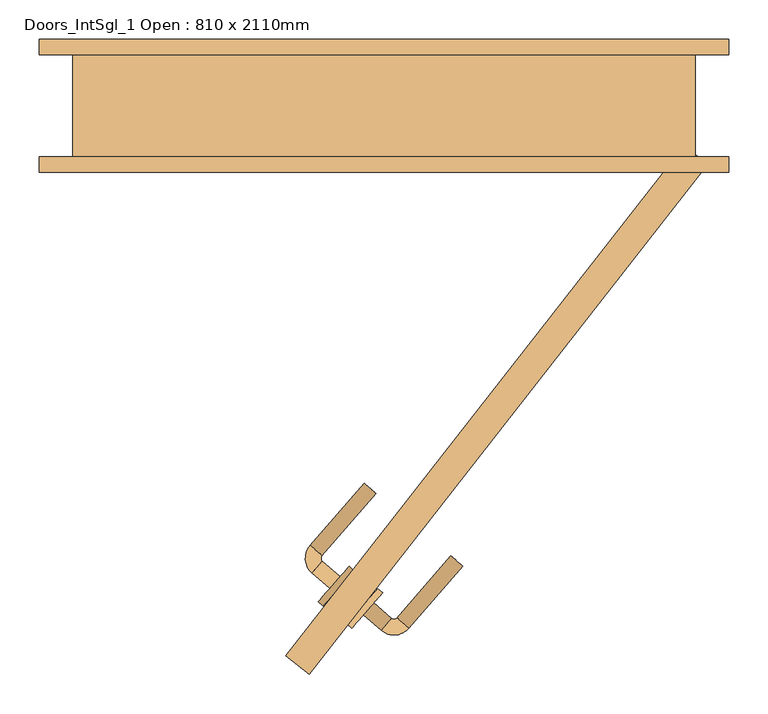
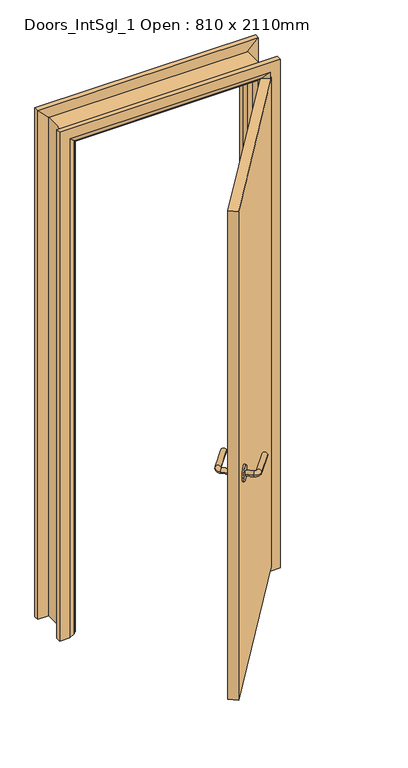
"""IFC4 building model written with IfcOpenShell, lengths in millimetres: door geometry, Doors_IntSgl_1 Open : 810 x 2110mm."""

import ifcopenshell
import ifcopenshell.guid

model = None  # the IFC model being written
_history = None  # IfcOwnerHistory: only IFC2X3 demands one
_inside = {}  # id of a spatial element -> (the spatial element, [elements in it])
_under = {}  # id of a project, library or spatial element -> (it, [spatial elements below it])
_declared = {}  # id of a project -> (the project, [libraries it declares])
_typed = {}  # id of a type object -> (the type object, [elements of that type])
_made_of = {}  # id of a material, layer set ... -> (it, [elements and type objects made of it])


def new_model(schema):
    """Start an empty IFC model of exactly this schema.

    Asked for "IFC4X3", IfcOpenShell would pick the latest addendum, in which some entities
    have other attributes; the version numbers below select the first issue.
    IFC2X3 requires an IfcOwnerHistory on every rooted entity: one is made here for all.
    """
    global model, _history
    if schema == "IFC4X3":
        model = ifcopenshell.file(schema_version=(4, 3, 0, 0))
    else:
        model = ifcopenshell.file(schema=schema)
    _inside.clear()
    _under.clear()
    _declared.clear()
    _typed.clear()
    _made_of.clear()
    _history = None
    if model.schema == "IFC2X3":
        org = make("IfcOrganization", Name="unknown")
        user = make(
            "IfcPersonAndOrganization",
            ThePerson=make("IfcPerson", FamilyName="unknown"),
            TheOrganization=org,
        )
        app = make(
            "IfcApplication",
            ApplicationDeveloper=org,
            Version="unknown",
            ApplicationFullName="unknown",
            ApplicationIdentifier="unknown",
        )
        _history = make(
            "IfcOwnerHistory",
            OwningUser=user,
            OwningApplication=app,
            ChangeAction="ADDED",
            CreationDate=0,
        )
    return model


def make(cls, **values):
    """One entity of the class cls with the attributes given. An attribute that is None is left unset."""
    return model.create_entity(
        cls, **{name: value for name, value in values.items() if value is not None}
    )


def rooted(cls, **values):
    """An entity with a GlobalId (a new one), such as an element, a storey or a relation."""
    return make(cls, GlobalId=ifcopenshell.guid.new(), OwnerHistory=_history, **values)


def si_unit(unit_type, name, prefix=None):
    """IfcSIUnit, for example si_unit("LENGTHUNIT", "METRE", prefix="MILLI")."""
    return make("IfcSIUnit", UnitType=unit_type, Prefix=prefix, Name=name)


def assignment(units):
    """IfcUnitAssignment: the units of a project."""
    return None if units is None else make("IfcUnitAssignment", Units=units)


def point(xyz):
    """IfcCartesianPoint."""
    return None if xyz is None else make("IfcCartesianPoint", Coordinates=xyz)


def direction(xyz):
    """IfcDirection."""
    return None if xyz is None else make("IfcDirection", DirectionRatios=xyz)


def frame(location, z_axis=None, x_axis=None):
    """IfcAxis2Placement3D, a coordinate frame: its origin and axes. An axis left out is left unset."""
    return make(
        "IfcAxis2Placement3D",
        Location=point(location),
        Axis=direction(z_axis),
        RefDirection=direction(x_axis),
    )


def frame_2d(location, x_axis=None):
    """IfcAxis2Placement2D, a coordinate frame in the plane: its origin and x axis."""
    return make(
        "IfcAxis2Placement2D", Location=point(location), RefDirection=direction(x_axis)
    )


def origin():
    """The frame at (0, 0, 0) with its axes left unset."""
    return frame((0.0, 0.0, 0.0))


def place(relative_to, where):
    """IfcLocalPlacement: puts the frame where relative to a parent placement (None: the world)."""
    return make(
        "IfcLocalPlacement", PlacementRelTo=relative_to, RelativePlacement=where
    )


def context(
    kind, dimensions, precision=None, world=None, true_north=None, identifier=None
):
    """IfcGeometricRepresentationContext, for example the 3D "Model" context."""
    return make(
        "IfcGeometricRepresentationContext",
        ContextIdentifier=identifier,
        ContextType=kind,
        CoordinateSpaceDimension=dimensions,
        Precision=precision,
        WorldCoordinateSystem=world,
        TrueNorth=true_north,
    )


def project(units=None, contexts=None):
    """IfcProject with its units and contexts."""
    return rooted(
        "IfcProject",
        Name="project",
        RepresentationContexts=contexts,
        UnitsInContext=assignment(units),
    )


def spatial(cls, under=None, at=None, **own):
    """A site, building, storey or space (cls), placed at a placement, below another one or the project."""
    s = rooted(cls, ObjectPlacement=at, **own)
    if under is not None:
        _under.setdefault(under.id(), (under, []))[1].append(s)
    return s


def polyline(points):
    """IfcPolyline through the points."""
    return make("IfcPolyline", Points=[point(p) for p in points])


def circle_curve(where, radius):
    """IfcCircle in the frame where."""
    return make("IfcCircle", Position=where, Radius=radius)


def ellipse_curve(where, semi_axis1, semi_axis2):
    """IfcEllipse in the frame where."""
    return make(
        "IfcEllipse", Position=where, SemiAxis1=semi_axis1, SemiAxis2=semi_axis2
    )


def trimmed(basis, trim1, trim2, sense, master):
    """IfcTrimmedCurve: the piece of a basis curve between two trims."""
    return make(
        "IfcTrimmedCurve",
        BasisCurve=basis,
        Trim1=trim1,
        Trim2=trim2,
        SenseAgreement=sense,
        MasterRepresentation=master,
    )


def segment(curve, same_sense, transition):
    """IfcCompositeCurveSegment."""
    return make(
        "IfcCompositeCurveSegment",
        Transition=transition,
        SameSense=same_sense,
        ParentCurve=curve,
    )


def composite_curve(segments, self_intersect=None):
    """IfcCompositeCurve: segments joined end to end."""
    return make("IfcCompositeCurve", Segments=segments, SelfIntersect=self_intersect)


def outline(outer, holes=None, kind="AREA"):
    """IfcArbitraryClosedProfileDef: a profile drawn as a closed curve; with holes, ...WithVoids."""
    if holes is None:
        return make("IfcArbitraryClosedProfileDef", ProfileType=kind, OuterCurve=outer)
    return make(
        "IfcArbitraryProfileDefWithVoids",
        ProfileType=kind,
        OuterCurve=outer,
        InnerCurves=holes,
    )


def extrude(swept, where, along, depth):
    """IfcExtrudedAreaSolid: the profile swept, set in the frame where, extruded along a direction by depth."""
    return make(
        "IfcExtrudedAreaSolid",
        SweptArea=swept,
        Position=where,
        ExtrudedDirection=direction(along),
        Depth=depth,
    )


def faces_of(points, faces, orient=None, outer=None):
    """IfcFace entities. A face is a list of loops; a loop is a list of indices into points, from 0.

    orient and outer hold one flag for each loop. By default every Orientation is true, the
    first loop of a face is its IfcFaceOuterBound and the others are IfcFaceBound.
    """
    made = []
    for i, loops in enumerate(faces):
        bounds = []
        for j, loop in enumerate(loops):
            is_outer = j == 0 if outer is None else outer[i][j]
            bounds.append(
                make(
                    "IfcFaceOuterBound" if is_outer else "IfcFaceBound",
                    Bound=make("IfcPolyLoop", Polygon=[points[k] for k in loop]),
                    Orientation=True if orient is None else orient[i][j],
                )
            )
        made.append(make("IfcFace", Bounds=bounds))
    return made


def faceted_brep(points, faces, orient=None, outer=None, voids=None):
    """IfcFacetedBrep: a solid bounded by flat faces; with voids (closed shells), ...WithVoids."""
    shared = [point(p) for p in points]
    hull = make("IfcClosedShell", CfsFaces=faces_of(shared, faces, orient, outer))
    if voids is None:
        return make("IfcFacetedBrep", Outer=hull)
    return make(
        "IfcFacetedBrepWithVoids",
        Outer=hull,
        Voids=[
            make(cls, CfsFaces=faces_of(shared, fs, o, b)) for cls, fs, o, b in voids
        ],
    )


def shape(context_of_items, identifier, shape_type, items):
    """IfcShapeRepresentation: the items that make up one representation, for example the "Body"."""
    return make(
        "IfcShapeRepresentation",
        ContextOfItems=context_of_items,
        RepresentationIdentifier=identifier,
        RepresentationType=shape_type,
        Items=items,
    )


def source(mapping_origin, context_of_items, identifier, shape_type, items):
    """IfcRepresentationMap: a shape defined once, which mapped items show again and again."""
    return make(
        "IfcRepresentationMap",
        MappingOrigin=mapping_origin,
        MappedRepresentation=shape(context_of_items, identifier, shape_type, items),
    )


def transform(
    local_origin,
    x_axis=None,
    y_axis=None,
    z_axis=None,
    scale=None,
    scale2=None,
    scale3=None,
    uniform=True,
):
    """IfcCartesianTransformationOperator3D, or its non-uniform kind. x_axis, y_axis, z_axis: its Axis1, 2, 3."""
    if uniform:
        return make(
            "IfcCartesianTransformationOperator3D",
            Axis1=direction(x_axis),
            Axis2=direction(y_axis),
            LocalOrigin=point(local_origin),
            Scale=scale,
            Axis3=direction(z_axis),
        )
    return make(
        "IfcCartesianTransformationOperator3DnonUniform",
        Axis1=direction(x_axis),
        Axis2=direction(y_axis),
        LocalOrigin=point(local_origin),
        Scale=scale,
        Axis3=direction(z_axis),
        Scale2=scale2,
        Scale3=scale3,
    )


def mapped(mapping_source, mapping_target):
    """IfcMappedItem: shows the shape of a source again, moved by a transform."""
    return make(
        "IfcMappedItem", MappingSource=mapping_source, MappingTarget=mapping_target
    )


def made_of(thing, what):
    """Note that an element or type object is made of a material, layer set ...; save() writes the relation."""
    if what is not None:
        _made_of.setdefault(what.id(), (what, []))[1].append(thing)
    return thing


def element(
    cls,
    number,
    at=None,
    inside=None,
    cuts=None,
    type_object=None,
    material=None,
    context=None,
    identifier="Body",
    shape_type=None,
    held_by="IfcProductDefinitionShape",
    body=None,
    shapes=None,
    **own,
):
    """One element of the class cls, such as IfcWall. Its Tag is "e" and its number.

    at: its placement. inside: the storey or other place that contains it. cuts: it is an
    opening in that element (IfcRelVoidsElement). A single representation is given by context,
    identifier, shape_type and body (its items); several are given by shapes. held_by: the class
    of the entity that holds the representations. save() writes the other relations.
    """
    e = rooted(cls, Tag="e%d" % number, ObjectPlacement=at, **own)
    if body is not None:
        shapes = [shape(context, identifier, shape_type, body)]
    if shapes is not None:
        e.Representation = make(held_by, Representations=shapes)
    if inside is not None:
        _inside.setdefault(inside.id(), (inside, []))[1].append(e)
    if cuts is not None:
        rooted(
            "IfcRelVoidsElement", RelatingBuildingElement=cuts, RelatedOpeningElement=e
        )
    if type_object is not None:
        _typed.setdefault(type_object.id(), (type_object, []))[1].append(e)
    return made_of(e, material)


def aggregate(whole, parts):
    """IfcRelAggregates: a whole, such as a stair, and the parts it consists of."""
    return rooted("IfcRelAggregates", RelatingObject=whole, RelatedObjects=parts)


def save(model, path):
    """Write the relations noted so far, then the file.

    IfcRelAggregates (storeys below a building ...), IfcRelContainedInSpatialStructure (elements
    in a storey), IfcRelDefinesByType, IfcRelAssociatesMaterial and IfcRelDeclares: one each for
    every whole, place, type object, material and project.
    """
    for whole, parts in _under.values():
        aggregate(whole, parts)
    for where, things in _inside.values():
        rooted(
            "IfcRelContainedInSpatialStructure",
            RelatedElements=things,
            RelatingStructure=where,
        )
    for kind, things in _typed.values():
        rooted("IfcRelDefinesByType", RelatedObjects=things, RelatingType=kind)
    for what, things in _made_of.values():
        rooted("IfcRelAssociatesMaterial", RelatedObjects=things, RelatingMaterial=what)
    for by, libraries in _declared.values():
        rooted("IfcRelDeclares", RelatingContext=by, RelatedDefinitions=libraries)
    model.write(path)


def plane_surface(at):
    """IfcPlane: the flat surface through the origin of the frame at, square to its z axis."""
    return make("IfcPlane", Position=at)


def cylinder_surface(at, radius):
    """IfcCylindricalSurface: all points at the distance radius from the z axis of the frame at."""
    return make("IfcCylindricalSurface", Position=at, Radius=radius)


def revolved_surface(curve, axis_point, axis_direction):
    """IfcSurfaceOfRevolution: the curve turned about the line through axis_point along axis_direction."""
    return make(
        "IfcSurfaceOfRevolution",
        SweptCurve=make("IfcArbitraryOpenProfileDef", ProfileType="CURVE", Curve=curve),
        AxisPosition=make("IfcAxis1Placement", Location=point(axis_point), Axis=direction(axis_direction)),
    )


def advanced_brep(points, edges, surfaces, faces):
    """IfcAdvancedBrep: a solid bounded by faces that lie on surfaces and meet in shared edges.

    An edge is (start, end): straight between two places in points (the first is 0);
    or (start, end, curve); or (start, end, curve, False) where it runs against its curve.
    A face is (place in surfaces, loops), or (place, loops, False) where it looks against
    its surface's normal. A loop lists edges by number (the first is 1), with a minus sign
    where the edge is run from its end to its start. The first loop is the outer one.
    """
    corners = [point(p) for p in points]
    vertices = [make("IfcVertexPoint", VertexGeometry=c) for c in corners]
    made = []
    for start, end, *more in edges:
        made.append(
            make(
                "IfcEdgeCurve",
                EdgeStart=vertices[start],
                EdgeEnd=vertices[end],
                EdgeGeometry=more[0] if more else make("IfcPolyline", Points=[corners[start], corners[end]]),
                SameSense=more[1] if len(more) > 1 else True,
            )
        )
    hull = []
    for where, loops, *sense in faces:
        bounds = []
        for j, loop in enumerate(loops):
            ring = [make("IfcOrientedEdge", EdgeElement=made[abs(k) - 1], Orientation=k > 0) for k in loop]
            bounds.append(
                make(
                    "IfcFaceOuterBound" if j == 0 else "IfcFaceBound",
                    Bound=make("IfcEdgeLoop", EdgeList=ring),
                    Orientation=True,
                )
            )
        hull.append(make("IfcAdvancedFace", Bounds=bounds, FaceSurface=surfaces[where], SameSense=sense[0] if sense else True))
    return make("IfcAdvancedBrep", Outer=make("IfcClosedShell", CfsFaces=hull))


def doors_intsgl_1_open_810_x_2110mm_3496c895(model_context):
    return source(origin(), model_context, "Body", "SolidModel", [
        advanced_brep(
        [(-69.1197704, -615.7042456, 900.0), (-55.9985898, -600.610054, 900.0), (-91.7610578, -596.0224748, 900.0), (-78.6398772, -580.9282832, 900.0), (-79.13313, -573.8744401, 900.0), (-94.2273216, -560.7532595, 900.0), (-25.3411235, -481.5087536, 900.0), (-10.2469319, -494.6299342, 900.0)],
        [
            (0, 1, circle_curve(frame((-62.5591801, -608.1571498, 900.0), z_axis=(0.7547095802227883, -0.6560590289904886, 0.0), x_axis=(0.6560590289904885, 0.7547095802227881, 0.0)), 10.0)),
            (1, 0, circle_curve(frame((-62.5591801, -608.1571498, 900.0), z_axis=(0.7547095802227883, -0.6560590289904886, 0.0), x_axis=(0.6560590289904885, 0.7547095802227881, 0.0)), 10.0)),
            (0, 2),
            (2, 3, circle_curve(frame((-85.2004675, -588.475379, 900.0), z_axis=(0.7547095802227883, -0.6560590289904886, 0.0), x_axis=(0.6560590289904885, 0.7547095802227881, 0.0)), 10.0)),
            (3, 1),
            (3, 2, circle_curve(frame((-85.2004675, -588.475379, 900.0), z_axis=(0.7547095802227883, -0.6560590289904886, 0.0), x_axis=(0.6560590289904885, 0.7547095802227881, 0.0)), 10.0)),
            (4, 3, circle_curve(frame((-75.3595821, -577.1547353, 900.0), z_axis=(0.0, 0.0, 1.0), x_axis=(-0.6560590289904885, -0.7547095802227881, 0.0)), 5.0)),
            (2, 5, circle_curve(frame((-75.3595821, -577.1547353, 900.0), z_axis=(0.0, 0.0, -1.0), x_axis=(-0.6560590289904885, -0.7547095802227881, 0.0)), 25.0)),
            (5, 4, circle_curve(frame((-86.6802258, -567.3138498, 900.0), z_axis=(-0.656059028990488, -0.7547095802227886, 0.0), x_axis=(0.7547095802227886, -0.656059028990488, 0.0)), 10.0)),
            (4, 5, circle_curve(frame((-86.6802258, -567.3138498, 900.0), z_axis=(-0.6560590289904857, -0.7547095802227904, 0.0), x_axis=(0.7547095802227904, -0.6560590289904857, 0.0)), 10.0)),
            (6, 7, circle_curve(frame((-17.7940277, -488.0693439, 900.0), z_axis=(0.6560590289904886, 0.7547095802227883, 0.0), x_axis=(0.7547095802227881, -0.6560590289904885, 0.0)), 10.0)),
            (7, 6, circle_curve(frame((-17.7940277, -488.0693439, 900.0), z_axis=(0.6560590289904886, 0.7547095802227883, 0.0), x_axis=(0.7547095802227881, -0.6560590289904885, 0.0)), 10.0)),
            (5, 6),
            (7, 4),
        ],
        [
            plane_surface(frame((-62.5591801, -608.1571498, 900.0), z_axis=(0.7547095802227883, -0.6560590289904886, 0.0), x_axis=(0.0, 0.0, 1.0))),
            cylinder_surface(frame((-62.5591801, -608.1571498, 900.0), z_axis=(0.7547095802227881, -0.6560590289904885, 0.0), x_axis=(0.6560590289904885, 0.7547095802227881, 0.0)), 10.0),
            revolved_surface(trimmed(ellipse_curve(frame((-85.2004675, -588.475379, 900.0), z_axis=(0.7547095802227881, -0.6560590289904885, 0.0), x_axis=(0.6560590289904885, 0.7547095802227881, 0.0)), 10.0, 10.0), [point((-91.7610578, -596.0224748, 900.0))], [point((-78.6398772, -580.9282832, 900.0))], True, "CARTESIAN"), (-75.3595821, -577.1547353, 900.0), (0.0, 0.0, -1.0)),
            revolved_surface(trimmed(ellipse_curve(frame((-85.2004675, -588.475379, 900.0), z_axis=(0.7547095802227881, -0.6560590289904885, 0.0), x_axis=(0.6560590289904885, 0.7547095802227881, 0.0)), 10.0, 10.0), [point((-78.6398772, -580.9282832, 900.0))], [point((-91.7610578, -596.0224748, 900.0))], True, "CARTESIAN"), (-75.3595821, -577.1547353, 900.0), (0.0, 0.0, -1.0)),
            plane_surface(frame((-17.7940277, -488.0693439, 900.0), z_axis=(0.6560590289904886, 0.7547095802227883, 0.0), x_axis=(0.0, 0.0, 1.0))),
            cylinder_surface(frame((-86.6802258, -567.3138498, 900.0), z_axis=(-0.6560590289904885, -0.7547095802227881, 0.0), x_axis=(0.7547095802227881, -0.6560590289904885, 0.0)), 10.0),
        ],
        [
            (0, [[1, 2]]),
            (1, [[-1, 3, 4, 5]]),
            (1, [[-2, -5, 6, -3]]),
            (2, [[7, -4, 8, 9]]),
            (3, [[-8, -6, -7, 10]]),
            (4, [[11, 12]]),
            (5, [[-9, 13, -12, 14]]),
            (5, [[-10, -14, -11, -13]]),
        ],
    ),
        extrude(outline(composite_curve([segment(trimmed(circle_curve(frame_2d((0.0, -30.0)), 30.0), [point((0.0, -60.0))], [point((0.0, 0.0))], False, "CARTESIAN"), True, "CONTINUOUS"), segment(trimmed(circle_curve(frame_2d((0.0, -30.0)), 30.0), [point((0.0, 0.0))], [point((0.0, -60.0))], False, "CARTESIAN"), True, "CONTINUOUS")], self_intersect=False)), frame((-38.4798801, -592.6511086, 900.0), z_axis=(-0.7547095802227883, 0.6560590289904886, 0.0), x_axis=(0.0, 0.0, 1.0)), (0.0, 0.0, 1.0), 8.0),
        advanced_brep(
        [(-26.2647476, -649.3053178, 900.0), (-13.143567, -634.2111262, 900.0), (9.4977204, -653.8928971, 900.0), (-3.6234602, -668.9870887, 900.0), (16.5515634, -653.3996443, 900.0), (31.645755, -666.5208249, 900.0), (100.5319531, -587.276319, 900.0), (85.4377615, -574.1551384, 900.0)],
        [
            (0, 1, circle_curve(frame((-19.7041573, -641.758222, 900.0), z_axis=(-0.7547095802227883, 0.6560590289904886, 0.0), x_axis=(0.6560590289904885, 0.7547095802227881, 0.0)), 10.0)),
            (1, 0, circle_curve(frame((-19.7041573, -641.758222, 900.0), z_axis=(-0.7547095802227883, 0.6560590289904886, 0.0), x_axis=(0.6560590289904885, 0.7547095802227881, 0.0)), 10.0)),
            (1, 2),
            (2, 3, circle_curve(frame((2.9371301, -661.4399929, 900.0), z_axis=(-0.7547095802227883, 0.6560590289904886, 0.0), x_axis=(0.6560590289904885, 0.7547095802227881, 0.0)), 10.0)),
            (3, 0),
            (3, 2, circle_curve(frame((2.9371301, -661.4399929, 900.0), z_axis=(-0.7547095802227883, 0.6560590289904886, 0.0), x_axis=(0.6560590289904885, 0.7547095802227881, 0.0)), 10.0)),
            (4, 5, circle_curve(frame((24.0986592, -659.9602346, 900.0), z_axis=(-0.6560590289904913, -0.7547095802227858, 0.0), x_axis=(-0.7547095802227858, 0.6560590289904913, 0.0)), 10.0)),
            (5, 3, circle_curve(frame((12.7780155, -650.1193492, 900.0), z_axis=(0.0, 0.0, -1.0), x_axis=(-0.6560590289904885, -0.7547095802227881, 0.0)), 25.0)),
            (2, 4, circle_curve(frame((12.7780155, -650.1193492, 900.0), z_axis=(0.0, 0.0, 1.0), x_axis=(-0.6560590289904885, -0.7547095802227881, 0.0)), 5.0)),
            (5, 4, circle_curve(frame((24.0986592, -659.9602346, 900.0), z_axis=(-0.6560590289904891, -0.7547095802227877, 0.0), x_axis=(-0.7547095802227877, 0.6560590289904891, 0.0)), 10.0)),
            (6, 7, circle_curve(frame((92.9848573, -580.7157287, 900.0), z_axis=(0.6560590289904886, 0.7547095802227883, 0.0), x_axis=(-0.7547095802227881, 0.6560590289904885, 0.0)), 10.0)),
            (7, 6, circle_curve(frame((92.9848573, -580.7157287, 900.0), z_axis=(0.6560590289904886, 0.7547095802227883, 0.0), x_axis=(-0.7547095802227881, 0.6560590289904885, 0.0)), 10.0)),
            (4, 7),
            (6, 5),
        ],
        [
            plane_surface(frame((-19.7041573, -641.758222, 900.0), z_axis=(-0.7547095802227883, 0.6560590289904886, 0.0), x_axis=(0.0, 0.0, 1.0))),
            cylinder_surface(frame((-19.7041573, -641.758222, 900.0), z_axis=(-0.7547095802227881, 0.6560590289904885, 0.0), x_axis=(0.6560590289904885, 0.7547095802227881, 0.0)), 10.0),
            revolved_surface(trimmed(ellipse_curve(frame((2.9371301, -661.4399929, 900.0), z_axis=(0.7547095802227881, -0.6560590289904885, 0.0), x_axis=(0.6560590289904885, 0.7547095802227881, 0.0)), 10.0, 10.0), [point((-3.6234602, -668.9870887, 900.0))], [point((9.4977204, -653.8928971, 900.0))], True, "CARTESIAN"), (12.7780155, -650.1193492, 900.0), (0.0, 0.0, -1.0)),
            revolved_surface(trimmed(ellipse_curve(frame((2.9371301, -661.4399929, 900.0), z_axis=(0.7547095802227881, -0.6560590289904885, 0.0), x_axis=(0.6560590289904885, 0.7547095802227881, 0.0)), 10.0, 10.0), [point((9.4977204, -653.8928971, 900.0))], [point((-3.6234602, -668.9870887, 900.0))], True, "CARTESIAN"), (12.7780155, -650.1193492, 900.0), (0.0, 0.0, -1.0)),
            plane_surface(frame((92.9848573, -580.7157287, 900.0), z_axis=(0.6560590289904886, 0.7547095802227883, 0.0), x_axis=(0.0, 0.0, 1.0))),
            cylinder_surface(frame((24.0986592, -659.9602346, 900.0), z_axis=(-0.6560590289904885, -0.7547095802227881, 0.0), x_axis=(-0.7547095802227881, 0.6560590289904885, 0.0)), 10.0),
        ],
        [
            (0, [[1, 2]]),
            (1, [[3, 4, 5, -2]]),
            (1, [[-5, 6, -3, -1]]),
            (2, [[7, 8, -4, 9]]),
            (3, [[10, -9, -6, -8]]),
            (4, [[11, 12]]),
            (5, [[13, -11, 14, -7]]),
            (5, [[-14, -12, -13, -10]]),
        ],
    ),
        extrude(outline(composite_curve([segment(trimmed(circle_curve(frame_2d((0.0, 30.0)), 30.0), [point((0.0, 60.0))], [point((0.0, 0.0))], False, "CARTESIAN"), True, "CONTINUOUS"), segment(trimmed(circle_curve(frame_2d((0.0, 30.0)), 30.0), [point((0.0, 0.0))], [point((0.0, 60.0))], False, "CARTESIAN"), True, "CONTINUOUS")], self_intersect=False)), frame((-1.662534, -621.0037086, 900.0), z_axis=(-0.7547095802227883, 0.6560590289904886, 0.0), x_axis=(0.0, 0.0, -1.0)), (0.0, 0.0, 1.0), 8.0),
        extrude(outline(polyline([(383.3995748, -51.0018026), (413.3439834, -74.3969387), (-95.1923952, -725.2938212), (-125.1368039, -701.8986851), (383.3995748, -51.0018026)])), frame((0.0, 0.0, 18.0), z_axis=(0.0, 0.0, 1.0), x_axis=(1.0, 0.0, 0.0)), (0.0, 0.0, 1.0), 2060.0),
        advanced_brep(
        [(440.0, -85.0, 0.0), (400.0, -85.0, 0.0), (374.0, -71.0, 0.0), (370.0, -65.0, 0.0), (440.0, -65.0, 0.0), (440.0, -65.0, 2145.0), (440.0, -85.0, 2145.0), (370.0, -65.0, 2075.0), (-370.0, -65.0, 2075.0), (-370.0, -65.0, 0.0), (-440.0, -65.0, 0.0), (-440.0, -65.0, 2145.0), (374.0, -71.0, 2079.0), (400.0, -85.0, 2105.0), (-440.0, -85.0, 2145.0), (-440.0, -85.0, 0.0), (-400.0, -85.0, 0.0), (-400.0, -85.0, 2105.0), (-374.0, -71.0, 0.0), (-374.0, -71.0, 2079.0)],
        [
            (0, 1),
            (1, 2),
            (2, 3, circle_curve(frame((378.0, -64.0, 0.0), z_axis=(0.0, 0.0, -1.0), x_axis=(1.0, 0.0, 0.0)), 8.0622577)),
            (3, 4),
            (4, 0),
            (4, 5),
            (5, 6),
            (6, 0),
            (3, 7),
            (7, 8),
            (8, 9),
            (9, 10),
            (10, 11),
            (11, 5),
            (2, 12),
            (12, 7, ellipse_curve(frame((378.0, -64.0, 2083.0), z_axis=(0.7071067811865475, 0.0, -0.7071067811865475), x_axis=(-0.7071067811865474, 0.0, -0.7071067811865476)), 11.4017543, 8.0622577)),
            (1, 13),
            (13, 12),
            (6, 14),
            (14, 15),
            (15, 16),
            (16, 17),
            (17, 13),
            (10, 15),
            (14, 11),
            (9, 18, circle_curve(frame((-378.0, -64.0, 0.0), z_axis=(0.0, 0.0, -1.0), x_axis=(-1.0, 0.0, 0.0)), 8.0622577)),
            (18, 16),
            (19, 18),
            (8, 19, ellipse_curve(frame((-378.0, -64.0, 2083.0), z_axis=(-0.7071067811865475, 0.0, -0.7071067811865475), x_axis=(-0.7071067811865474, 0.0, 0.7071067811865476)), 11.4017543, 8.0622577)),
            (19, 17),
            (12, 19),
        ],
        [
            plane_surface(frame((370.0, -65.0, 0.0), z_axis=(0.0, 0.0, -1.0), x_axis=(0.0, 1.0, 0.0))),
            plane_surface(frame((440.0, -85.0, 0.0), z_axis=(1.0, 0.0, 0.0), x_axis=(0.0, 0.0, 1.0))),
            plane_surface(frame((440.0, -65.0, 0.0), z_axis=(0.0, 1.0, 0.0), x_axis=(0.0, 0.0, 1.0))),
            cylinder_surface(frame((378.0, -64.0, 0.0), z_axis=(0.0, 0.0, -1.0), x_axis=(1.0, 0.0, 0.0)), 8.0622577),
            plane_surface(frame((374.0, -71.0, 0.0), z_axis=(-0.4740998230350126, -0.880471099922178, 0.0), x_axis=(0.0, 0.0, 1.0))),
            plane_surface(frame((400.0, -85.0, 0.0), z_axis=(0.0, -1.0, 0.0), x_axis=(0.0, 0.0, 1.0))),
            plane_surface(frame((-440.0, -85.0, 2145.0), z_axis=(-1.0, 0.0, 0.0), x_axis=(0.0, 0.0, -1.0))),
            plane_surface(frame((-370.0, -65.0, 0.0), z_axis=(0.0, 0.0, -1.0), x_axis=(0.0, 1.0, 0.0))),
            cylinder_surface(frame((-378.0, -64.0, 2075.0), z_axis=(0.0, 0.0, 1.0), x_axis=(-1.0, 0.0, 0.0)), 8.0622577),
            plane_surface(frame((-374.0, -71.0, 2079.0), z_axis=(0.47409982303501824, -0.8804710999221749, 0.0), x_axis=(0.0, 0.0, -1.0))),
            plane_surface(frame((440.0, -85.0, 2145.0), z_axis=(0.0, 0.0, 1.0), x_axis=(-1.0, 0.0, 0.0))),
            cylinder_surface(frame((370.0, -64.0, 2083.0), z_axis=(1.0, 0.0, 0.0), x_axis=(0.0, 0.0, 1.0)), 8.0622577),
            plane_surface(frame((374.0, -71.0, 2079.0), z_axis=(0.0, -0.8804710999221764, -0.4740998230350154), x_axis=(-1.0, 0.0, 0.0))),
        ],
        [
            (0, [[1, 2, 3, 4, 5]]),
            (1, [[6, 7, 8, -5]]),
            (2, [[9, 10, 11, 12, 13, 14, -6, -4]]),
            (3, [[15, 16, -9, -3]]),
            (4, [[17, 18, -15, -2]]),
            (5, [[-8, 19, 20, 21, 22, 23, -17, -1]]),
            (6, [[-13, 24, -20, 25]]),
            (7, [[-24, -12, 26, 27, -21]]),
            (8, [[28, -26, -11, 29]]),
            (9, [[-22, -27, -28, 30]]),
            (10, [[-14, -25, -19, -7]]),
            (11, [[31, -29, -10, -16]]),
            (12, [[-23, -30, -31, -18]]),
        ],
    ),
        extrude(outline(polyline([(0.0, -346.0), (2051.0, -346.0), (2051.0, 346.0), (0.0, 346.0), (0.0, 365.0), (2070.0, 365.0), (2070.0, -365.0), (0.0, -365.0), (0.0, -346.0)])), frame((0.0, -25.0, 0.0), z_axis=(0.0, 1.0, 0.0), x_axis=(0.0, 0.0, 1.0)), (0.0, 0.0, 1.0), 32.0),
        advanced_brep(
        [(-440.0, 85.0, 0.0), (-400.0, 85.0, 0.0), (-374.0, 71.0, 0.0), (-370.0, 65.0, 0.0), (-440.0, 65.0, 0.0), (-440.0, 65.0, 2145.0), (-440.0, 85.0, 2145.0), (-370.0, 65.0, 2075.0), (-374.0, 71.0, 2079.0), (-400.0, 85.0, 2105.0), (440.0, 85.0, 0.0), (440.0, 65.0, 0.0), (370.0, 65.0, 0.0), (374.0, 71.0, 0.0), (400.0, 85.0, 0.0), (440.0, 85.0, 2145.0), (400.0, 85.0, 2105.0), (374.0, 71.0, 2079.0), (370.0, 65.0, 2075.0), (440.0, 65.0, 2145.0)],
        [
            (0, 1),
            (1, 2),
            (2, 3, circle_curve(frame((-378.0, 64.0, 0.0), z_axis=(0.0, 0.0, -1.0), x_axis=(-1.0, 0.0, 0.0)), 8.0622577)),
            (3, 4),
            (4, 0),
            (4, 5),
            (5, 6),
            (6, 0),
            (3, 7),
            (7, 5),
            (2, 8),
            (8, 7, ellipse_curve(frame((-378.0, 64.0, 2083.0), z_axis=(-0.7071067811865475, 0.0, -0.7071067811865475), x_axis=(0.7071067811865474, 0.0, -0.7071067811865476)), 11.4017543, 8.0622577)),
            (1, 9),
            (9, 8),
            (6, 9),
            (10, 11),
            (11, 12),
            (12, 13, circle_curve(frame((378.0, 64.0, 0.0), z_axis=(0.0, 0.0, -1.0), x_axis=(1.0, 0.0, 0.0)), 8.0622577)),
            (13, 14),
            (14, 10),
            (15, 10),
            (14, 16),
            (16, 15),
            (13, 17),
            (17, 16),
            (12, 18),
            (18, 17, ellipse_curve(frame((378.0, 64.0, 2083.0), z_axis=(0.7071067811865475, 0.0, -0.7071067811865475), x_axis=(0.7071067811865474, 0.0, 0.7071067811865476)), 11.4017543, 8.0622577)),
            (11, 19),
            (19, 18),
            (15, 19),
            (5, 19),
            (15, 6),
            (7, 18),
            (8, 17),
            (9, 16),
        ],
        [
            plane_surface(frame((-370.0, 137.8010989, 0.0), z_axis=(0.0, 0.0, -1.0), x_axis=(1.0, 0.0, 0.0))),
            plane_surface(frame((-440.0, 85.0, 0.0), z_axis=(-1.0, 0.0, 0.0), x_axis=(0.0, 0.0, 1.0))),
            plane_surface(frame((-440.0, 65.0, 0.0), z_axis=(0.0, -1.0, 0.0), x_axis=(0.0, 0.0, 1.0))),
            cylinder_surface(frame((-378.0, 64.0, 0.0), z_axis=(0.0, 0.0, -1.0), x_axis=(-1.0, 0.0, 0.0)), 8.0622577),
            plane_surface(frame((-374.0, 71.0, 0.0), z_axis=(0.4740998230350183, 0.8804710999221749, 0.0), x_axis=(0.0, 0.0, 1.0))),
            plane_surface(frame((-400.0, 85.0, 0.0), z_axis=(0.0, 1.0, 0.0), x_axis=(0.0, 0.0, 1.0))),
            plane_surface(frame((370.0, 137.8010989, 0.0), z_axis=(0.0, 0.0, -1.0), x_axis=(-1.0, 0.0, 0.0))),
            plane_surface(frame((400.0, 85.0, 2105.0), z_axis=(0.0, 1.0, 0.0), x_axis=(0.0, 0.0, -1.0))),
            plane_surface(frame((374.0, 71.0, 2079.0), z_axis=(-0.4740998230350183, 0.8804710999221749, 0.0), x_axis=(0.0, 0.0, -1.0))),
            cylinder_surface(frame((378.0, 64.0, 2075.0), z_axis=(0.0, 0.0, 1.0), x_axis=(1.0, 0.0, 0.0)), 8.0622577),
            plane_surface(frame((440.0, 65.0, 2145.0), z_axis=(0.0, -1.0, 0.0), x_axis=(0.0, 0.0, -1.0))),
            plane_surface(frame((440.0, 85.0, 2145.0), z_axis=(1.0, 0.0, 0.0), x_axis=(0.0, 0.0, -1.0))),
            plane_surface(frame((-440.0, 85.0, 2145.0), z_axis=(0.0, 0.0, 1.0), x_axis=(1.0, 0.0, 0.0))),
            plane_surface(frame((-440.0, 65.0, 2145.0), z_axis=(0.0, -1.0, 0.0), x_axis=(1.0, 0.0, 0.0))),
            cylinder_surface(frame((-370.0, 64.0, 2083.0), z_axis=(-1.0, 0.0, 0.0), x_axis=(0.0, 0.0, 1.0)), 8.0622577),
            plane_surface(frame((-374.0, 71.0, 2079.0), z_axis=(0.0, 0.8804710999221749, -0.4740998230350183), x_axis=(1.0, 0.0, 0.0))),
            plane_surface(frame((-400.0, 85.0, 2105.0), z_axis=(0.0, 1.0, 0.0), x_axis=(1.0, 0.0, 0.0))),
        ],
        [
            (0, [[1, 2, 3, 4, 5]]),
            (1, [[6, 7, 8, -5]]),
            (2, [[9, 10, -6, -4]]),
            (3, [[11, 12, -9, -3]]),
            (4, [[13, 14, -11, -2]]),
            (5, [[-8, 15, -13, -1]]),
            (6, [[16, 17, 18, 19, 20]]),
            (7, [[21, -20, 22, 23]]),
            (8, [[-22, -19, 24, 25]]),
            (9, [[-24, -18, 26, 27]]),
            (10, [[-26, -17, 28, 29]]),
            (11, [[-28, -16, -21, 30]]),
            (12, [[31, -30, 32, -7]]),
            (13, [[33, -29, -31, -10]]),
            (14, [[34, -27, -33, -12]]),
            (15, [[35, -25, -34, -14]]),
            (16, [[-32, -23, -35, -15]]),
        ],
    ),
        faceted_brep([(-365.0, -65.0, 0.0), (-397.0, -65.0, 0.0), (-397.0, 65.0, 0.0), (-365.0, 65.0, 0.0), (-365.0, 65.0, 2070.0), (-365.0, -65.0, 2070.0), (-397.0, 65.0, 2102.0), (-397.0, -65.0, 2102.0), (365.0, -65.0, 0.0), (365.0, 65.0, 0.0), (397.0, 65.0, 0.0), (397.0, -65.0, 0.0), (365.0, -65.0, 2070.0), (397.0, -65.0, 2102.0), (397.0, 65.0, 2102.0), (365.0, 65.0, 2070.0)], [[[0, 1, 2, 3]], [[3, 4, 5, 0]], [[2, 6, 4, 3]], [[1, 7, 6, 2]], [[0, 5, 7, 1]], [[8, 9, 10, 11]], [[12, 8, 11, 13]], [[13, 11, 10, 14]], [[14, 10, 9, 15]], [[15, 9, 8, 12]], [[4, 15, 12, 5]], [[6, 14, 15, 4]], [[7, 13, 14, 6]], [[5, 12, 13, 7]]]),
    ])


if __name__ == "__main__":
    model = new_model("IFC4")
    model_context = context("Model", 3, world=origin())
    ifc_project = project(units=[si_unit("LENGTHUNIT", "METRE", prefix="MILLI")], contexts=[model_context])
    site = spatial("IfcSite", under=ifc_project)
    building = spatial("IfcBuilding", under=site)
    placement = place(None, origin())
    doors_intsgl_1_open_810_x_2110mm_shape = doors_intsgl_1_open_810_x_2110mm_3496c895(model_context)
    element("IfcDoor", 1, ObjectType="Doors_IntSgl_1 Open : 810 x 2110mm", at=placement, inside=building, context=model_context, shape_type="MappedRepresentation", body=[
        mapped(doors_intsgl_1_open_810_x_2110mm_shape, transform((0.0, 0.0, 0.0), x_axis=(1.0, 0.0, 0.0), y_axis=(0.0, 1.0, 0.0), z_axis=(0.0, 0.0, 1.0))),
    ])
    save(model, "model.ifc")

# Revit data of these elements
# Type "Doors_IntSgl_1 Open : 810 x 2110mm"
#   Type Mark = "69"
#   Type Comments = "Internal Single"
#   Operation = "SingleSwingRight"
#   Manufacturer = "Revit"
#   Keynote = "L20"
#   Description = "Internal Single Door"
#   Analytic Construction = "Metal"
#   UnderCut = 8 mm
#   Tolerance = 2 mm
#   Thickness = 38 mm
#   Thermal Resistance (R) = 0.270117 (m²·K)/W
#   Structural Tolerance = 8 mm
#   StopDepth = 32 mm
#   Stop Thickness = 19 mm
#   Rough Width = 810 mm
#   Rough Height = 2110 mm
#   Height to Top Lock Rail = 1000 mm
#   Heat Transfer Coefficient (U) = 3.7021 W/(m²·K)
#   Handle Z Distance = 900 mm
#   Handle X Distance = 75 mm
#   Frame Thickness = 32 mm
#   Door Panel Width = 726 mm
#   Door Panel Thickness = 38 mm
#   Door Panel Offset = 0 mm
#   Height = 2110 mm
#   Width = 810 mm
#   Door Panel Height = 2060 mm
#   Architrave Setback = 5 mm
#   Vis - Ironmongery = yes
#   Material Ironmongery = Door - Handle
#   Material Frame = Door - Frame/Mullion (1)
#   Material Door = Door - Panel
#   Material Architrave = Door - Architrave
#   Visual Light Transmittance = 0
#   Solar Heat Gain Coefficient = 0
#   Function = (empty or 0)
#   Wall Closure = (empty or 0)
# Element 1 (IfcDoor, "Doors_IntSgl_1 Open : 810 x 2110mm")
#   Materials on its faces: "Door - Architrave", "Door - Handle", "Door - Frame/Mullion (1)", "Door - Panel"
# Materials
#   "Door - Handle": class "Miscellaneous", colour RGB 0 0 0, transparency 0, Keynote = "P21"
#   "Door - Frame/Mullion (1)": class "Wood", colour RGB 212 179 113, transparency 0, Keynote = "L20", Cost = 0
#   "Door - Panel": class "Wood", colour RGB 210 159 95, transparency 0, Keynote = "L20"
#   "Door - Architrave": class "Wood", colour RGB 154 90 5, transparency 0, Keynote = "P20"
